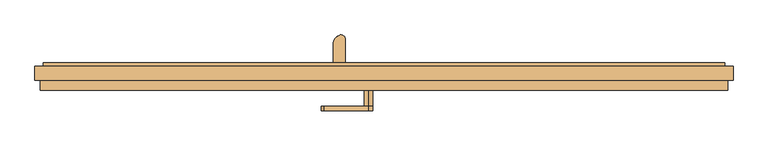
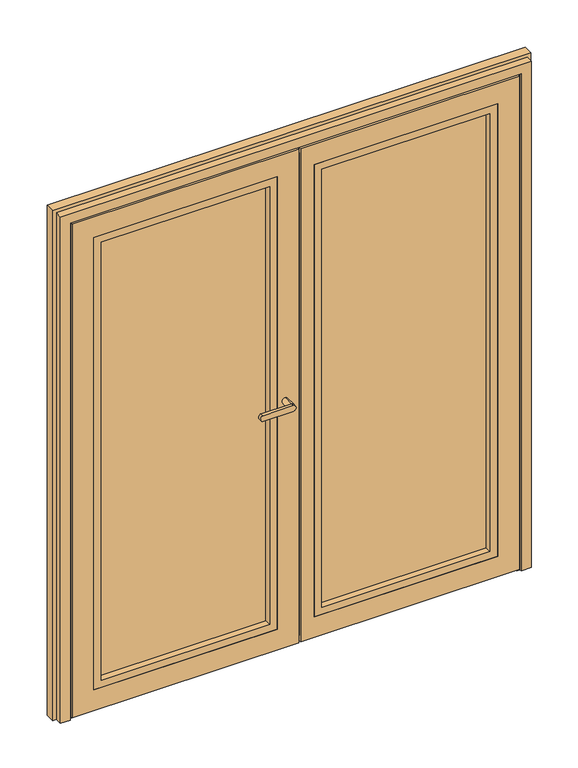
"""IFC4 building model written with IfcOpenShell, lengths in millimetres: door geometry, Schueco_FWS_ADS-75-BL-SimplySmart_inw_Family-02 : FWS SI insert unit."""

from ifc_helpers import new_model, si_unit, point, frame, frame_2d, origin, place, context, project, spatial, polyline, circle_curve, ellipse_curve, trimmed, segment, composite_curve, outline, extrude, faceted_brep, source, transform, mapped, element, save
from ifc_brep_helpers import plane_surface, cylinder_surface, extruded_surface, advanced_brep


def door_aeff8a81(model_context):
    return source(origin(), model_context, "Body", "SolidModel", [
        faceted_brep([(893.0, -57.5000065, 8.0), (893.0, -57.5000065, 2093.0), (893.0, -66.0002823, 2093.0), (893.0, -66.0002823, 8.0), (19.5, -66.0002823, 8.0), (19.5, -57.5000065, 8.0), (19.5, -57.5000065, 30.0), (871.0, -57.5000065, 30.0), (871.0, -57.5000065, 2071.0), (19.5, -57.5000065, 2071.0), (19.5, -57.5000065, 2093.0), (19.5, -66.0002823, 2093.0), (73.5, -66.0002823, 95.0), (73.5, -66.0002823, 2006.0), (806.0, -66.0002823, 2006.0), (806.0, -66.0002823, 95.0), (806.0, -2.0002726, 2006.0), (806.0, -2.0002726, 95.0), (73.5, -2.0002726, 95.0), (73.5, -2.0002726, 2006.0), (105.5, -2.0002726, 127.0), (105.5, -2.0002726, 1974.0), (774.0, -2.0002726, 1974.0), (774.0, -2.0002726, 127.0), (774.0, 8.9997177, 1974.0), (774.0, 8.9997177, 127.0), (105.5, 8.9997177, 127.0), (105.5, 8.9997177, 1974.0), (861.0, 8.9997177, 40.0), (-12.5, 8.9997177, 40.0), (-12.5, 8.9997177, 2061.0), (861.0, 8.9997177, 2061.0), (861.0, 0.4997603, 2061.0), (861.0, 0.4997603, 40.0), (8.5, 0.4997603, 40.0), (-12.5, 0.4997603, 40.0), (8.5, 0.4997603, 30.0), (8.5, 0.4997603, 2061.0), (8.5, 0.4997603, 2071.0), (871.0, 0.4997603, 2071.0), (871.0, 0.4997603, 30.0), (8.5, -57.5000065, 30.0), (8.5, -57.5000065, 2071.0), (-12.5, 0.4997603, 2061.0)], [[[0, 1, 2, 3]], [[3, 4, 5, 0]], [[0, 5, 6, 7, 8, 9, 10, 1]], [[2, 11, 4, 3], [12, 13, 14, 15]], [[15, 14, 16, 17]], [[17, 18, 12, 15]], [[18, 19, 13, 12]], [[17, 16, 19, 18], [20, 21, 22, 23]], [[23, 22, 24, 25]], [[25, 26, 20, 23]], [[26, 27, 21, 20]], [[28, 29, 30, 31], [25, 24, 27, 26]], [[28, 31, 32, 33]], [[33, 34, 35, 29, 28]], [[36, 34, 33, 32, 37, 38, 39, 40]], [[40, 39, 8, 7]], [[7, 6, 41, 36, 40]], [[41, 42, 38, 37, 34, 36]], [[1, 10, 11, 2]], [[19, 16, 14, 13]], [[27, 24, 22, 21]], [[31, 30, 43, 37, 32]], [[42, 9, 8, 39, 38]], [[6, 5, 4, 11, 10, 9]], [[35, 43, 30, 29]], [[35, 34, 37, 43]], [[9, 42, 41, 6]]]),
        extrude(outline(polyline([(95.0, 73.5), (95.0, 806.0), (2006.0, 806.0), (2006.0, 73.5), (95.0, 73.5)]), holes=[polyline([(125.0, 776.0), (125.0, 103.5), (1976.0, 103.5), (1976.0, 776.0), (125.0, 776.0)])]), frame((0.0, -66.0002823, 0.0), z_axis=(0.0, 1.0, 0.0), x_axis=(0.0, 0.0, 1.0)), (0.0, 0.0, 1.0), 26.0000097),
        extrude(outline(polyline([(73.5, -40.0002726), (73.5, -2.0002726), (806.0, -2.0002726), (806.0, -40.0002726), (73.5, -40.0002726)])), frame((0.0, 0.0, 95.0), z_axis=(0.0, 0.0, 1.0), x_axis=(1.0, 0.0, 0.0)), (0.0, 0.0, 1.0), 1911.0),
        extrude(outline(composite_curve([segment(polyline([(-39.1486683, 30.0), (-17.8439358, 30.0), (-17.8439358, 4.0204884)]), True, "CONTINUOUS"), segment(trimmed(circle_curve(frame_2d((-28.496302, 16.1220734)), 16.1220739), [point((-17.8439358, 4.0204884))], [point((-39.1486683, 4.0204884))], False, "CARTESIAN"), True, "CONTINUOUS"), segment(polyline([(-39.1486683, 4.0204884), (-39.1486683, 30.0)]), True, "CONTINUOUS")], self_intersect=False)), frame((8.5, 0.0, 0.0), z_axis=(1.0, 0.0, 0.0), x_axis=(0.0, 1.0, 0.0)), (0.0, 0.0, 1.0), 862.5),
        extrude(outline(polyline([(861.0, 0.4997603), (-12.5, 0.4997603), (-12.5, 8.9997177), (861.0, 8.9997177), (861.0, 0.4997603)])), frame((0.0, 0.0, 8.0), z_axis=(0.0, 0.0, 1.0), x_axis=(1.0, 0.0, 0.0)), (0.0, 0.0, 1.0), 32.0),
        extrude(outline(composite_curve([segment(polyline([(-139.1672968, 8.9997177), (-139.1672968, 59.1618682)]), True, "CONTINUOUS"), segment(trimmed(circle_curve(frame_2d((-111.9888791, 59.1618682)), 27.1784177), [point((-139.1672968, 59.1618682))], [point((-121.5259747, 84.6120194))], False, "CARTESIAN"), True, "CONTINUOUS"), segment(trimmed(circle_curve(frame_2d((-117.4484738, 73.7310321)), 11.6198924), [point((-121.5259747, 84.6120194))], [point((-105.8285814, 73.7310321))], False, "CARTESIAN"), True, "CONTINUOUS"), segment(polyline([(-105.8285814, 73.7310321), (-105.8285814, 8.9997177), (-139.1672968, 8.9997177)]), True, "CONTINUOUS")], self_intersect=False)), frame((0.0, 0.0, 2036.9340013), z_axis=(0.0, 0.0, 1.0), x_axis=(1.0, 0.0, 0.0)), (0.0, 0.0, 1.0), 4.0),
        extrude(outline(polyline([(-139.1672968, 12.9997177), (-105.8285814, 12.9997177), (-105.8285814, 8.9997177), (-139.1672968, 8.9997177), (-139.1672968, 12.9997177)])), frame((0.0, 0.0, 2006.9340013), z_axis=(0.0, 0.0, 1.0), x_axis=(1.0, 0.0, 0.0)), (0.0, 0.0, 1.0), 30.0),
        extrude(outline(polyline([(-139.1672968, 12.9997177), (-105.8285814, 12.9997177), (-105.8285814, 8.9997177), (-139.1672968, 8.9997177), (-139.1672968, 12.9997177)])), frame((0.0, 0.0, 56.9340013), z_axis=(0.0, 0.0, 1.0), x_axis=(1.0, 0.0, 0.0)), (0.0, 0.0, 1.0), 30.0),
        extrude(outline(composite_curve([segment(polyline([(-139.1672968, 8.9997177), (-139.1672968, 59.1618682)]), True, "CONTINUOUS"), segment(trimmed(circle_curve(frame_2d((-111.9888791, 59.1618682)), 27.1784177), [point((-139.1672968, 59.1618682))], [point((-121.5259747, 84.6120194))], False, "CARTESIAN"), True, "CONTINUOUS"), segment(trimmed(circle_curve(frame_2d((-117.4484738, 73.7310321)), 11.6198924), [point((-121.5259747, 84.6120194))], [point((-105.8285814, 73.7310321))], False, "CARTESIAN"), True, "CONTINUOUS"), segment(polyline([(-105.8285814, 73.7310321), (-105.8285814, 8.9997177), (-139.1672968, 8.9997177)]), True, "CONTINUOUS")], self_intersect=False)), frame((0.0, 0.0, 52.9340013), z_axis=(0.0, 0.0, 1.0), x_axis=(1.0, 0.0, 0.0)), (0.0, 0.0, 1.0), 4.0),
        advanced_brep(
        [(-109.7828972, 57.5977179, 2036.9340013), (-135.2170493, 72.2821425, 2036.9340013), (-109.7828972, 57.5977179, 56.9340013), (-135.2170493, 72.2821425, 56.9340013)],
        [
            (0, 1, ellipse_curve(frame((-122.4999732, 64.9399302, 2036.9340013), z_axis=(0.0, 0.0, 1.0000000000000002), x_axis=(0.5000002582658958, 0.866025254674503, 0.0)), 21.5840887, 14.6844171)),
            (1, 0, ellipse_curve(frame((-122.4999732, 64.9399302, 2036.9340013), z_axis=(0.0, 0.0, 1.0000000000000002), x_axis=(0.5000002582658958, 0.866025254674503, 0.0)), 21.5840887, 14.6844171)),
            (2, 3, ellipse_curve(frame((-122.4999732, 64.9399302, 56.9340013), z_axis=(0.0, 0.0, -1.0000000000000002), x_axis=(-0.866025254674503, 0.5000002582658958, 0.0)), 14.6844171, 21.5840887)),
            (3, 2, ellipse_curve(frame((-122.4999732, 64.9399302, 56.9340013), z_axis=(0.0, 0.0, -1.0000000000000002), x_axis=(-0.866025254674503, 0.5000002582658958, 0.0)), 14.6844171, 21.5840887)),
            (0, 2),
            (3, 1),
        ],
        [
            plane_surface(frame((-135.2170493, 72.2821425, 2036.9340013), z_axis=(0.0, 0.0, 1.0000000000000002), x_axis=(0.5000002582658958, 0.866025254674503, 0.0))),
            plane_surface(frame((-135.2170493, 72.2821425, 56.9340013), z_axis=(0.0, 0.0, -1.0000000000000002), x_axis=(-0.5000002582658958, -0.866025254674503, 0.0))),
            extruded_surface(trimmed(ellipse_curve(frame((-122.4999732, 64.9399302, 56.9340013), z_axis=(0.0, 0.0, -1.0000000000000002), x_axis=(-0.866025254674503, 0.5000002582658958, 0.0)), 14.6844171, 21.5840887), [point((-135.2170493, 72.2821425, 56.9340013))], [point((-109.7828972, 57.5977179, 56.9340013))], True, "CARTESIAN"), (0.0, 0.0, -1980.0), 1980.0),
            extruded_surface(trimmed(ellipse_curve(frame((-122.4999732, 64.9399302, 56.9340013), z_axis=(0.0, 0.0, -1.0000000000000002), x_axis=(-0.866025254674503, 0.5000002582658958, 0.0)), 14.6844171, 21.5840887), [point((-109.7828972, 57.5977179, 56.9340013))], [point((-135.2170493, 72.2821425, 56.9340013))], True, "CARTESIAN"), (0.0, 0.0, -1980.0), 1980.0),
        ],
        [
            (0, [[1, 2]]),
            (1, [[3, 4]]),
            (2, [[5, -4, 6, -1]]),
            (3, [[-6, -3, -5, -2]]),
        ],
    ),
        advanced_brep(
        [(-42.4999732, -122.0002518, 1038.0113692), (-42.4999732, -122.0002518, 1061.9886308), (-164.1617658, -122.0002518, 1061.9886308), (-164.1617658, -122.0002518, 1038.0113692), (-42.4999732, -109.5001648, 1061.9886308), (-42.4999732, -109.5001648, 1038.0113692), (-164.1617658, -109.5001648, 1038.0113692), (-164.1617658, -109.5001648, 1061.9886308), (-42.4999732, -66.0002823, 1038.0113692), (-42.4999732, -66.0002823, 1061.9886308)],
        [
            (0, 1, circle_curve(frame((-42.4999732, -122.0002518, 1050.0), z_axis=(0.0, -1.0, 0.0), x_axis=(0.0, 0.0, 1.0)), 11.9886308)),
            (1, 2),
            (2, 3, ellipse_curve(frame((-164.1617658, -122.0002518, 1050.0), z_axis=(0.0, -1.0, 0.0), x_axis=(0.0, 0.0, -1.0)), 11.9886308, 7.9050795)),
            (3, 0),
            (4, 5, circle_curve(frame((-42.4999732, -109.5001648, 1050.0), z_axis=(0.0, -1.0, 0.0), x_axis=(0.0, 0.0, 1.0)), 11.9886308)),
            (5, 6),
            (6, 7, ellipse_curve(frame((-164.1617658, -109.5001648, 1050.0), z_axis=(0.0, 1.0, 0.0), x_axis=(0.0, 0.0, -1.0)), 11.9886308, 7.9050795)),
            (7, 4),
            (3, 6),
            (5, 0),
            (2, 7),
            (1, 4),
            (5, 4, circle_curve(frame((-42.4999732, -109.5001648, 1050.0), z_axis=(0.0, -1.0, 0.0), x_axis=(0.0, 0.0, 1.0)), 11.9886308)),
            (8, 9, circle_curve(frame((-42.4999732, -66.0002823, 1050.0), z_axis=(0.0, 1.0, 0.0), x_axis=(0.0, 0.0, 1.0)), 11.9886308)),
            (9, 8, circle_curve(frame((-42.4999732, -66.0002823, 1050.0), z_axis=(0.0, 1.0, 0.0), x_axis=(0.0, 0.0, 1.0)), 11.9886308)),
            (8, 5),
            (4, 9),
        ],
        [
            plane_surface(frame((-164.1617658, -122.0002518, 1038.0113692), z_axis=(0.0, -1.0, 0.0), x_axis=(-1.0, 0.0, 0.0))),
            plane_surface(frame((-164.1617658, -109.5001648, 1038.0113692), z_axis=(0.0, 1.0, 0.0), x_axis=(1.0, 0.0, 0.0))),
            plane_surface(frame((-42.4999732, -122.0002518, 1038.0113692), z_axis=(0.0, 0.0, -1.0), x_axis=(0.0, 1.0, 0.0))),
            extruded_surface(trimmed(ellipse_curve(frame((-164.1617658, -109.5001648, 1050.0), z_axis=(0.0, 1.0, 0.0), x_axis=(0.0, 0.0, -1.0)), 11.9886308, 7.9050795), [point((-164.1617658, -109.5001648, 1038.0113692))], [point((-164.1617658, -109.5001648, 1061.9886308))], True, "CARTESIAN"), (0.0, 12.500086999999994, 0.0), 12.500086999999994),
            plane_surface(frame((-164.1617658, -122.0002518, 1061.9886308), z_axis=(0.0, 0.0, 1.0), x_axis=(0.0, 1.0, 0.0))),
            cylinder_surface(frame((-42.4999732, -109.5001648, 1050.0), z_axis=(0.0, -1.0, 0.0), x_axis=(0.0, 0.0, 1.0)), 11.9886308),
            plane_surface(frame((-42.4999732, -66.0002823, 1061.9886308), z_axis=(0.0, 1.0, 0.0), x_axis=(-1.0, 0.0, 0.0))),
            cylinder_surface(frame((-42.4999732, -66.0002823, 1050.0), z_axis=(0.0, -1.0, 0.0), x_axis=(0.0, 0.0, 1.0)), 11.9886308),
        ],
        [
            (0, [[1, 2, 3, 4]]),
            (1, [[5, 6, 7, 8]]),
            (2, [[9, -6, 10, -4]]),
            (3, [[11, -7, -9, -3]]),
            (4, [[12, -8, -11, -2]]),
            (5, [[-10, 13, -12, -1]]),
            (6, [[14, 15]]),
            (7, [[16, -5, 17, -14]]),
            (7, [[-17, -13, -16, -15]]),
        ],
    ),
        faceted_brep([(-892.9999732, -57.5000065, 8.0), (-892.9999732, -66.0002823, 8.0), (-892.9999732, -66.0002823, 2093.0), (-892.9999732, -57.5000065, 2093.0), (12.5000268, -57.5000065, 8.0), (12.5000268, -66.0002823, 8.0), (12.5000268, -57.5000065, 2093.0), (-870.9999732, -57.5000065, 30.0), (-9.4999732, -57.5000065, 30.0), (-9.4999732, -57.5000065, 2071.0), (-870.9999732, -57.5000065, 2071.0), (12.5000268, -66.0002823, 2093.0), (-74.4999732, -66.0002823, 95.0), (-805.9999732, -66.0002823, 95.0), (-805.9999732, -66.0002823, 2006.0), (-74.4999732, -66.0002823, 2006.0), (-805.9999732, -2.0002726, 95.0), (-805.9999732, -2.0002726, 2006.0), (-74.4999732, -2.0002726, 95.0), (-74.4999732, -2.0002726, 2006.0), (-106.4999732, -2.0002726, 127.0), (-773.9999732, -2.0002726, 127.0), (-773.9999732, -2.0002726, 1974.0), (-106.4999732, -2.0002726, 1974.0), (-773.9999732, 8.9997177, 127.0), (-773.9999732, 8.9997177, 1974.0), (-106.4999732, 8.9997177, 127.0), (-106.4999732, 8.9997177, 1974.0), (-19.4999732, 8.9997177, 2061.0), (-19.4999732, 8.9997177, 40.0), (-29.4999732, 8.9997177, 40.0), (-860.9999732, 8.9997177, 40.0), (-860.9999732, 8.9997177, 2061.0), (-29.4999732, 8.9997177, 2061.0), (-860.9999732, 0.4997603, 40.0), (-860.9999732, 0.4997603, 2061.0), (-19.4999732, 0.4997603, 40.0), (-29.4999732, 0.4997603, 40.0), (-19.4999732, 0.4997603, 2061.0), (-9.4999732, 0.4997603, 30.0), (-870.9999732, 0.4997603, 30.0), (-870.9999732, 0.4997603, 2071.0), (-9.4999732, 0.4997603, 2071.0), (-29.4999732, 0.4997603, 2061.0)], [[[0, 1, 2, 3]], [[1, 0, 4, 5]], [[4, 0, 3, 6], [7, 8, 9, 10]], [[5, 4, 6, 11]], [[1, 5, 11, 2], [12, 13, 14, 15]], [[13, 16, 17, 14]], [[16, 13, 12, 18]], [[18, 12, 15, 19]], [[16, 18, 19, 17], [20, 21, 22, 23]], [[21, 24, 25, 22]], [[24, 21, 20, 26]], [[26, 20, 23, 27]], [[28, 29, 30, 31, 32, 33], [24, 26, 27, 25]], [[31, 34, 35, 32]], [[34, 31, 30, 29, 36, 37]], [[36, 29, 28, 38]], [[39, 40, 41, 42], [36, 38, 43, 35, 34, 37]], [[40, 7, 10, 41]], [[7, 40, 39, 8]], [[8, 39, 42, 9]], [[11, 6, 3, 2]], [[19, 15, 14, 17]], [[27, 23, 22, 25]], [[38, 28, 33, 32, 35, 43]], [[9, 42, 41, 10]]]),
        extrude(outline(polyline([(95.0, -74.4999732), (2006.0, -74.4999732), (2006.0, -805.9999732), (95.0, -805.9999732), (95.0, -74.4999732)]), holes=[polyline([(125.0, -775.9999732), (1976.0, -775.9999732), (1976.0, -104.4999732), (125.0, -104.4999732), (125.0, -775.9999732)])]), frame((0.0, -66.0002823, 0.0), z_axis=(0.0, 1.0, 0.0), x_axis=(0.0, 0.0, 1.0)), (0.0, 0.0, 1.0), 26.0000097),
        extrude(outline(polyline([(-74.4999732, -40.0002726), (-805.9999732, -40.0002726), (-805.9999732, -2.0002726), (-74.4999732, -2.0002726), (-74.4999732, -40.0002726)])), frame((0.0, 0.0, 95.0), z_axis=(0.0, 0.0, 1.0), x_axis=(1.0, 0.0, 0.0)), (0.0, 0.0, 1.0), 1911.0),
        extrude(outline(composite_curve([segment(polyline([(-39.1486683, 30.0), (-17.8439358, 30.0), (-17.8439358, 4.0204884)]), True, "CONTINUOUS"), segment(trimmed(circle_curve(frame_2d((-28.496302, 16.1220734)), 16.1220739), [point((-17.8439358, 4.0204884))], [point((-39.1486683, 4.0204884))], False, "CARTESIAN"), True, "CONTINUOUS"), segment(polyline([(-39.1486683, 4.0204884), (-39.1486683, 30.0)]), True, "CONTINUOUS")], self_intersect=False)), frame((-870.9999732, 0.0, 0.0), z_axis=(1.0, 0.0, 0.0), x_axis=(0.0, 1.0, 0.0)), (0.0, 0.0, 1.0), 861.5),
        extrude(outline(polyline([(-860.9999732, 0.4997603), (-860.9999732, 8.9997177), (-19.4999732, 8.9997177), (-19.4999732, 0.4997603), (-860.9999732, 0.4997603)])), frame((0.0, 0.0, 8.0), z_axis=(0.0, 0.0, 1.0), x_axis=(1.0, 0.0, 0.0)), (0.0, 0.0, 1.0), 32.0),
        faceted_brep([(930.999943, 8.9997177, 2130.999943), (930.999943, 0.0, 2130.999943), (930.999943, 0.0, 0.0), (930.999943, 8.9997177, 0.0), (-954.0, 0.0, 0.0), (-954.0, 0.0, 2154.0), (954.0, 0.0, 2154.0), (954.0, 0.0, 0.0), (-930.999943, 0.0, 2130.999943), (-930.999943, 0.0, 0.0), (954.0, -38.0, 0.0), (940.0, -38.0, 0.0), (940.0, -66.0002823, 0.0), (899.9999732, -66.0002823, 0.0), (899.9999732, -57.5000065, 0.0), (888.4999732, -57.5000065, 0.0), (888.4999732, 0.4997603, 0.0), (867.9999732, 0.4997603, 0.0), (867.9999732, 8.9997177, 0.0), (-867.9999732, 8.9997177, 0.0), (-930.999943, 8.9997177, 0.0), (-930.999943, 8.9997177, 2130.999943), (867.9999732, 8.9997177, 2067.9999732), (-867.9999732, 8.9997177, 2067.9999732), (899.9999732, -66.0002823, 2099.9999732), (899.9999732, -57.5000065, 2099.9999732), (-899.9999732, -57.5000065, 0.0), (-888.4999732, -57.5000065, 0.0), (-888.4999732, -57.5000065, 2088.4999732), (888.4999732, -57.5000065, 2088.4999732), (-899.9999732, -57.5000065, 2099.9999732), (-940.0, -66.0002823, 0.0), (-899.9999732, -66.0002823, 0.0), (-899.9999732, -66.0002823, 2099.9999732), (940.0, -66.0002823, 2140.0), (-940.0, -66.0002823, 2140.0), (940.0, -38.0, 2140.0), (-954.0, -38.0, 0.0), (-940.0, -38.0, 0.0), (-940.0, -38.0, 2140.0), (954.0, -38.0, 2154.0), (-954.0, -38.0, 2154.0), (-867.9999732, 0.4997603, 0.0), (-888.4999732, 0.4997603, 0.0), (867.9999732, 0.4997603, 2067.9999732), (-867.9999732, 0.4997603, 2067.9999732), (888.4999732, 0.4997603, 2088.4999732), (-888.4999732, 0.4997603, 2088.4999732)], [[[0, 1, 2, 3]], [[4, 5, 6, 7, 2, 1, 8, 9]], [[3, 2, 7, 10, 11, 12, 13, 14, 15, 16, 17, 18]], [[19, 20, 21, 0, 3, 18, 22, 23]], [[24, 25, 14, 13]], [[26, 27, 28, 29, 15, 14, 25, 30]], [[31, 32, 33, 24, 13, 12, 34, 35]], [[34, 12, 11, 36]], [[37, 38, 39, 36, 11, 10, 40, 41]], [[4, 9, 20, 19, 42, 43, 27, 26, 32, 31, 38, 37]], [[20, 9, 8, 21]], [[18, 17, 44, 22]], [[42, 19, 23, 45]], [[32, 26, 30, 33]], [[31, 35, 39, 38]], [[4, 37, 41, 5]], [[6, 40, 10, 7]], [[43, 42, 45, 44, 17, 16, 46, 47]], [[16, 15, 29, 46]], [[27, 43, 47, 28]], [[21, 8, 1, 0]], [[33, 30, 25, 24]], [[35, 34, 36, 39]], [[23, 22, 44, 45]], [[5, 41, 40, 6]], [[47, 46, 29, 28]]]),
    ])


if __name__ == "__main__":
    model = new_model("IFC4")
    model_context = context("Model", 3, world=origin())
    ifc_project = project(units=[si_unit("LENGTHUNIT", "METRE", prefix="MILLI")], contexts=[model_context])
    site = spatial("IfcSite", under=ifc_project)
    building = spatial("IfcBuilding", under=site)
    placement = place(None, origin())
    door_shape = door_aeff8a81(model_context)
    element("IfcDoor", 1, ObjectType="Schueco_FWS_ADS-75-BL-SimplySmart_inw_Family-02 : FWS SI insert unit", at=placement, inside=building, context=model_context, shape_type="MappedRepresentation", body=[
        mapped(door_shape, transform((0.0, 0.0, 0.0), x_axis=(1.0, 0.0, 0.0), y_axis=(0.0, 1.0, 0.0), z_axis=(0.0, 0.0, 1.0))),
    ])
    save(model, "model.ifc")

# Revit data of these elements
# Type "Schueco_FWS_ADS-75-BL-SimplySmart_inw_Family-02 : FWS SI insert unit"
#   Type Mark = "29"
#   __NOTE__ = "Data describes the optimum values of the entire system. The properites of a selected design option have to be determined on an individual basis!"
#   Wind load resistance = "Class C3"
#   Watertightness = "Class E750"
#   Thermal insulation = "Uf = 1.6 W/(m²K)"
#   Sound insulation = "..."
#   Schueco thermal insulation standard = "Highly thermally insulated"
#   Opening type = "Inward-opening, Flush-fitted"
#   Model = "Schueco ADS 75 BL SimplySmart"
#   Mechanical loading = "..."
#   Maximum leaf width in mm = "1400"
#   Maximum leaf weight in kg = "200"
#   Maximum leaf height in mm = "3000"
#   Material = "Aluminium"
#   Long term functionality = "..."
#   Construction Type = "Door, double-leaf, inward-opening"
#   Manufacturer = "Schueco International KG"
#   Glazing data = "Triple glazing 38mm"
#   Façade insert unit = "yes"
#   Family creation date = "08.2017"
#   Description = "Schueco Aluminium Door System (ADS)"
#   Burglar resistance = "Class RC 2"
#   Areas of use = "Public buildings, Residential buildings, Side entrance"
#   Analytic Construction = "<None>"
#   Air permeability = "Class 4"
#   Width [instance default] = 949.001 mm
#   Leaf opening angle [instance default] = 0.00°
#   IOf_T = 38 mm
#   Height [instance default] = 1923.399 mm
#   Glazing area [instance default] = 0.609384 m²
#   F2_W [instance default] = 475.5 mm
#   F1_W [instance default] = 474.5 mm
#   Distance from bottom to handles [instance default] = 1050 mm
#   Clear opening width [instance default] = 777.001 mm
#   Active leaf width = 1100 mm
#   Standard threshold = no
#   Low level threshold = yes
#   Handles = yes
#   FWS SI insert unit = yes
#   FWS HI insert unit = no
#   All fields of identical width = yes
#   Glass = none
#   Frame = Alu
#   Fittings = none
# Element 1 (IfcDoor, "Schueco_FWS_ADS-75-BL-SimplySmart_inw_Family-02 : FWS SI insert unit")
#   Width = 1908 mm
#   Height = 2154 mm
#   Glazing area = 2.46759 m²
#   F2_W = 955 mm
#   F1_W = 954 mm
#   Clear opening width = 1736 mm
#   Materials on its faces: "Alu", "Glass"
# Materials
#   "Alu": class "Glas", colour RGB 140 140 140, transparency 0
#   "Glass": class "Glass", colour RGB 128 128 255, transparency 0.75, Description = "Soda Lime Glass", Cost = 0
